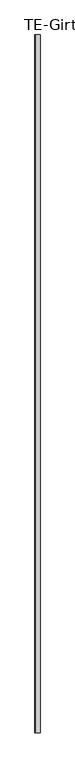
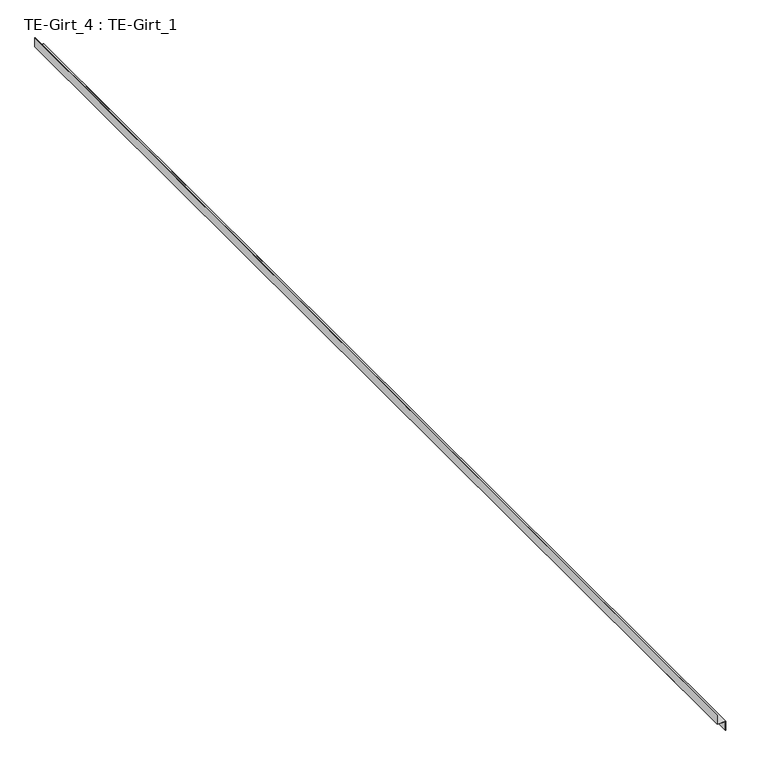
"""IFC4 building model written with IfcOpenShell, lengths in millimetres: proxy geometry, TE-Girt_4 : TE-Girt_1."""

from ifc_helpers import new_model, si_unit, frame, origin, place, context, project, spatial, polyline, outline, extrude, source, transform, mapped, element, save


def te_girt_4_te_girt_1_95d38daf(model_context):
    return source(origin(), model_context, "Body", "SweptSolid", [
        extrude(outline(polyline([(844.55, 590353.5520246), (844.55, 590319.5364427), (881.7570313, 590319.5364427), (881.7570313, 590318.6434739), (843.6570313, 590318.6434739), (843.6570313, 590352.6590559), (806.45, 590352.6590559), (806.45, 590353.5520246), (844.55, 590353.5520246)])), frame((0.0, -536417.5913841, 0.0), z_axis=(0.0, 1.0, 0.0), x_axis=(0.0, 0.0, 1.0)), (0.0, 0.0, 1.0), 4778.375),
    ])


if __name__ == "__main__":
    model = new_model("IFC4")
    model_context = context("Model", 3, world=origin())
    ifc_project = project(units=[si_unit("LENGTHUNIT", "METRE", prefix="MILLI")], contexts=[model_context])
    site = spatial("IfcSite", under=ifc_project)
    building = spatial("IfcBuilding", under=site)
    placement = place(None, origin())
    te_girt_4_te_girt_1_shape = te_girt_4_te_girt_1_95d38daf(model_context)
    element("IfcBuildingElementProxy", 1, Name="TE-Girt_4 : TE-Girt_1", ObjectType="TE-Girt_4 : TE-Girt_1", at=placement, inside=building, context=model_context, shape_type="MappedRepresentation", body=[
        mapped(te_girt_4_te_girt_1_shape, transform((0.0, 0.0, 0.0), x_axis=(1.0, 0.0, 0.0), y_axis=(0.0, 1.0, 0.0), z_axis=(0.0, 0.0, 1.0))),
    ])
    save(model, "model.ifc")

# Revit data of these elements
# Element 1 (IfcBuildingElementProxy, "TE-Girt_4 : TE-Girt_1")
#   Materials on its faces: "Z-FURRING, COLD-FORMED GALV."
# Materials
#   "Z-FURRING, COLD-FORMED GALV.": class "Generic", colour RGB 143 142 141, transparency 0, Cost = 0
